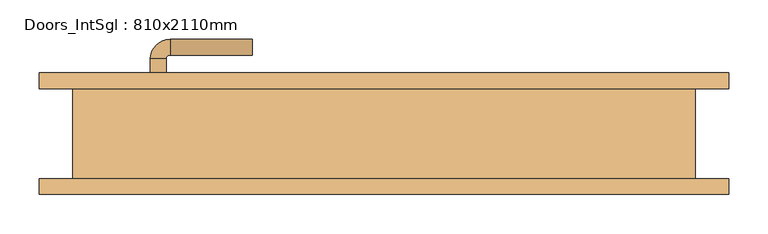
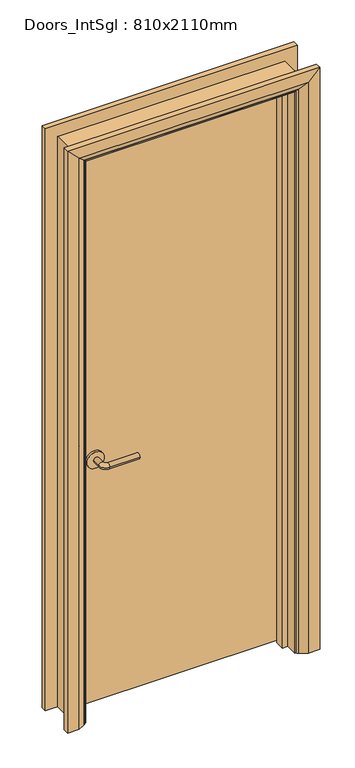
"""IFC4 building model written with IfcOpenShell, lengths in millimetres: door geometry, Doors_IntSgl : 810x2110mm."""

import ifcopenshell
import ifcopenshell.guid

model = None  # the IFC model being written
_history = None  # IfcOwnerHistory: only IFC2X3 demands one
_inside = {}  # id of a spatial element -> (the spatial element, [elements in it])
_under = {}  # id of a project, library or spatial element -> (it, [spatial elements below it])
_declared = {}  # id of a project -> (the project, [libraries it declares])
_typed = {}  # id of a type object -> (the type object, [elements of that type])
_made_of = {}  # id of a material, layer set ... -> (it, [elements and type objects made of it])


def new_model(schema):
    """Start an empty IFC model of exactly this schema.

    Asked for "IFC4X3", IfcOpenShell would pick the latest addendum, in which some entities
    have other attributes; the version numbers below select the first issue.
    IFC2X3 requires an IfcOwnerHistory on every rooted entity: one is made here for all.
    """
    global model, _history
    if schema == "IFC4X3":
        model = ifcopenshell.file(schema_version=(4, 3, 0, 0))
    else:
        model = ifcopenshell.file(schema=schema)
    _inside.clear()
    _under.clear()
    _declared.clear()
    _typed.clear()
    _made_of.clear()
    _history = None
    if model.schema == "IFC2X3":
        org = make("IfcOrganization", Name="unknown")
        user = make(
            "IfcPersonAndOrganization",
            ThePerson=make("IfcPerson", FamilyName="unknown"),
            TheOrganization=org,
        )
        app = make(
            "IfcApplication",
            ApplicationDeveloper=org,
            Version="unknown",
            ApplicationFullName="unknown",
            ApplicationIdentifier="unknown",
        )
        _history = make(
            "IfcOwnerHistory",
            OwningUser=user,
            OwningApplication=app,
            ChangeAction="ADDED",
            CreationDate=0,
        )
    return model


def make(cls, **values):
    """One entity of the class cls with the attributes given. An attribute that is None is left unset."""
    return model.create_entity(
        cls, **{name: value for name, value in values.items() if value is not None}
    )


def rooted(cls, **values):
    """An entity with a GlobalId (a new one), such as an element, a storey or a relation."""
    return make(cls, GlobalId=ifcopenshell.guid.new(), OwnerHistory=_history, **values)


def si_unit(unit_type, name, prefix=None):
    """IfcSIUnit, for example si_unit("LENGTHUNIT", "METRE", prefix="MILLI")."""
    return make("IfcSIUnit", UnitType=unit_type, Prefix=prefix, Name=name)


def assignment(units):
    """IfcUnitAssignment: the units of a project."""
    return None if units is None else make("IfcUnitAssignment", Units=units)


def point(xyz):
    """IfcCartesianPoint."""
    return None if xyz is None else make("IfcCartesianPoint", Coordinates=xyz)


def direction(xyz):
    """IfcDirection."""
    return None if xyz is None else make("IfcDirection", DirectionRatios=xyz)


def frame(location, z_axis=None, x_axis=None):
    """IfcAxis2Placement3D, a coordinate frame: its origin and axes. An axis left out is left unset."""
    return make(
        "IfcAxis2Placement3D",
        Location=point(location),
        Axis=direction(z_axis),
        RefDirection=direction(x_axis),
    )


def frame_2d(location, x_axis=None):
    """IfcAxis2Placement2D, a coordinate frame in the plane: its origin and x axis."""
    return make(
        "IfcAxis2Placement2D", Location=point(location), RefDirection=direction(x_axis)
    )


def origin():
    """The frame at (0, 0, 0) with its axes left unset."""
    return frame((0.0, 0.0, 0.0))


def place(relative_to, where):
    """IfcLocalPlacement: puts the frame where relative to a parent placement (None: the world)."""
    return make(
        "IfcLocalPlacement", PlacementRelTo=relative_to, RelativePlacement=where
    )


def context(
    kind, dimensions, precision=None, world=None, true_north=None, identifier=None
):
    """IfcGeometricRepresentationContext, for example the 3D "Model" context."""
    return make(
        "IfcGeometricRepresentationContext",
        ContextIdentifier=identifier,
        ContextType=kind,
        CoordinateSpaceDimension=dimensions,
        Precision=precision,
        WorldCoordinateSystem=world,
        TrueNorth=true_north,
    )


def project(units=None, contexts=None):
    """IfcProject with its units and contexts."""
    return rooted(
        "IfcProject",
        Name="project",
        RepresentationContexts=contexts,
        UnitsInContext=assignment(units),
    )


def spatial(cls, under=None, at=None, **own):
    """A site, building, storey or space (cls), placed at a placement, below another one or the project."""
    s = rooted(cls, ObjectPlacement=at, **own)
    if under is not None:
        _under.setdefault(under.id(), (under, []))[1].append(s)
    return s


def polyline(points):
    """IfcPolyline through the points."""
    return make("IfcPolyline", Points=[point(p) for p in points])


def circle_curve(where, radius):
    """IfcCircle in the frame where."""
    return make("IfcCircle", Position=where, Radius=radius)


def ellipse_curve(where, semi_axis1, semi_axis2):
    """IfcEllipse in the frame where."""
    return make(
        "IfcEllipse", Position=where, SemiAxis1=semi_axis1, SemiAxis2=semi_axis2
    )


def trimmed(basis, trim1, trim2, sense, master):
    """IfcTrimmedCurve: the piece of a basis curve between two trims."""
    return make(
        "IfcTrimmedCurve",
        BasisCurve=basis,
        Trim1=trim1,
        Trim2=trim2,
        SenseAgreement=sense,
        MasterRepresentation=master,
    )


def segment(curve, same_sense, transition):
    """IfcCompositeCurveSegment."""
    return make(
        "IfcCompositeCurveSegment",
        Transition=transition,
        SameSense=same_sense,
        ParentCurve=curve,
    )


def composite_curve(segments, self_intersect=None):
    """IfcCompositeCurve: segments joined end to end."""
    return make("IfcCompositeCurve", Segments=segments, SelfIntersect=self_intersect)


def outline(outer, holes=None, kind="AREA"):
    """IfcArbitraryClosedProfileDef: a profile drawn as a closed curve; with holes, ...WithVoids."""
    if holes is None:
        return make("IfcArbitraryClosedProfileDef", ProfileType=kind, OuterCurve=outer)
    return make(
        "IfcArbitraryProfileDefWithVoids",
        ProfileType=kind,
        OuterCurve=outer,
        InnerCurves=holes,
    )


def extrude(swept, where, along, depth):
    """IfcExtrudedAreaSolid: the profile swept, set in the frame where, extruded along a direction by depth."""
    return make(
        "IfcExtrudedAreaSolid",
        SweptArea=swept,
        Position=where,
        ExtrudedDirection=direction(along),
        Depth=depth,
    )


def faces_of(points, faces, orient=None, outer=None):
    """IfcFace entities. A face is a list of loops; a loop is a list of indices into points, from 0.

    orient and outer hold one flag for each loop. By default every Orientation is true, the
    first loop of a face is its IfcFaceOuterBound and the others are IfcFaceBound.
    """
    made = []
    for i, loops in enumerate(faces):
        bounds = []
        for j, loop in enumerate(loops):
            is_outer = j == 0 if outer is None else outer[i][j]
            bounds.append(
                make(
                    "IfcFaceOuterBound" if is_outer else "IfcFaceBound",
                    Bound=make("IfcPolyLoop", Polygon=[points[k] for k in loop]),
                    Orientation=True if orient is None else orient[i][j],
                )
            )
        made.append(make("IfcFace", Bounds=bounds))
    return made


def faceted_brep(points, faces, orient=None, outer=None, voids=None):
    """IfcFacetedBrep: a solid bounded by flat faces; with voids (closed shells), ...WithVoids."""
    shared = [point(p) for p in points]
    hull = make("IfcClosedShell", CfsFaces=faces_of(shared, faces, orient, outer))
    if voids is None:
        return make("IfcFacetedBrep", Outer=hull)
    return make(
        "IfcFacetedBrepWithVoids",
        Outer=hull,
        Voids=[
            make(cls, CfsFaces=faces_of(shared, fs, o, b)) for cls, fs, o, b in voids
        ],
    )


def shape(context_of_items, identifier, shape_type, items):
    """IfcShapeRepresentation: the items that make up one representation, for example the "Body"."""
    return make(
        "IfcShapeRepresentation",
        ContextOfItems=context_of_items,
        RepresentationIdentifier=identifier,
        RepresentationType=shape_type,
        Items=items,
    )


def source(mapping_origin, context_of_items, identifier, shape_type, items):
    """IfcRepresentationMap: a shape defined once, which mapped items show again and again."""
    return make(
        "IfcRepresentationMap",
        MappingOrigin=mapping_origin,
        MappedRepresentation=shape(context_of_items, identifier, shape_type, items),
    )


def transform(
    local_origin,
    x_axis=None,
    y_axis=None,
    z_axis=None,
    scale=None,
    scale2=None,
    scale3=None,
    uniform=True,
):
    """IfcCartesianTransformationOperator3D, or its non-uniform kind. x_axis, y_axis, z_axis: its Axis1, 2, 3."""
    if uniform:
        return make(
            "IfcCartesianTransformationOperator3D",
            Axis1=direction(x_axis),
            Axis2=direction(y_axis),
            LocalOrigin=point(local_origin),
            Scale=scale,
            Axis3=direction(z_axis),
        )
    return make(
        "IfcCartesianTransformationOperator3DnonUniform",
        Axis1=direction(x_axis),
        Axis2=direction(y_axis),
        LocalOrigin=point(local_origin),
        Scale=scale,
        Axis3=direction(z_axis),
        Scale2=scale2,
        Scale3=scale3,
    )


def mapped(mapping_source, mapping_target):
    """IfcMappedItem: shows the shape of a source again, moved by a transform."""
    return make(
        "IfcMappedItem", MappingSource=mapping_source, MappingTarget=mapping_target
    )


def made_of(thing, what):
    """Note that an element or type object is made of a material, layer set ...; save() writes the relation."""
    if what is not None:
        _made_of.setdefault(what.id(), (what, []))[1].append(thing)
    return thing


def element(
    cls,
    number,
    at=None,
    inside=None,
    cuts=None,
    type_object=None,
    material=None,
    context=None,
    identifier="Body",
    shape_type=None,
    held_by="IfcProductDefinitionShape",
    body=None,
    shapes=None,
    **own,
):
    """One element of the class cls, such as IfcWall. Its Tag is "e" and its number.

    at: its placement. inside: the storey or other place that contains it. cuts: it is an
    opening in that element (IfcRelVoidsElement). A single representation is given by context,
    identifier, shape_type and body (its items); several are given by shapes. held_by: the class
    of the entity that holds the representations. save() writes the other relations.
    """
    e = rooted(cls, Tag="e%d" % number, ObjectPlacement=at, **own)
    if body is not None:
        shapes = [shape(context, identifier, shape_type, body)]
    if shapes is not None:
        e.Representation = make(held_by, Representations=shapes)
    if inside is not None:
        _inside.setdefault(inside.id(), (inside, []))[1].append(e)
    if cuts is not None:
        rooted(
            "IfcRelVoidsElement", RelatingBuildingElement=cuts, RelatedOpeningElement=e
        )
    if type_object is not None:
        _typed.setdefault(type_object.id(), (type_object, []))[1].append(e)
    return made_of(e, material)


def aggregate(whole, parts):
    """IfcRelAggregates: a whole, such as a stair, and the parts it consists of."""
    return rooted("IfcRelAggregates", RelatingObject=whole, RelatedObjects=parts)


def save(model, path):
    """Write the relations noted so far, then the file.

    IfcRelAggregates (storeys below a building ...), IfcRelContainedInSpatialStructure (elements
    in a storey), IfcRelDefinesByType, IfcRelAssociatesMaterial and IfcRelDeclares: one each for
    every whole, place, type object, material and project.
    """
    for whole, parts in _under.values():
        aggregate(whole, parts)
    for where, things in _inside.values():
        rooted(
            "IfcRelContainedInSpatialStructure",
            RelatedElements=things,
            RelatingStructure=where,
        )
    for kind, things in _typed.values():
        rooted("IfcRelDefinesByType", RelatedObjects=things, RelatingType=kind)
    for what, things in _made_of.values():
        rooted("IfcRelAssociatesMaterial", RelatedObjects=things, RelatingMaterial=what)
    for by, libraries in _declared.values():
        rooted("IfcRelDeclares", RelatingContext=by, RelatedDefinitions=libraries)
    model.write(path)


def plane_surface(at):
    """IfcPlane: the flat surface through the origin of the frame at, square to its z axis."""
    return make("IfcPlane", Position=at)


def cylinder_surface(at, radius):
    """IfcCylindricalSurface: all points at the distance radius from the z axis of the frame at."""
    return make("IfcCylindricalSurface", Position=at, Radius=radius)


def revolved_surface(curve, axis_point, axis_direction):
    """IfcSurfaceOfRevolution: the curve turned about the line through axis_point along axis_direction."""
    return make(
        "IfcSurfaceOfRevolution",
        SweptCurve=make("IfcArbitraryOpenProfileDef", ProfileType="CURVE", Curve=curve),
        AxisPosition=make("IfcAxis1Placement", Location=point(axis_point), Axis=direction(axis_direction)),
    )


def advanced_brep(points, edges, surfaces, faces):
    """IfcAdvancedBrep: a solid bounded by faces that lie on surfaces and meet in shared edges.

    An edge is (start, end): straight between two places in points (the first is 0);
    or (start, end, curve); or (start, end, curve, False) where it runs against its curve.
    A face is (place in surfaces, loops), or (place, loops, False) where it looks against
    its surface's normal. A loop lists edges by number (the first is 1), with a minus sign
    where the edge is run from its end to its start. The first loop is the outer one.
    """
    corners = [point(p) for p in points]
    vertices = [make("IfcVertexPoint", VertexGeometry=c) for c in corners]
    made = []
    for start, end, *more in edges:
        made.append(
            make(
                "IfcEdgeCurve",
                EdgeStart=vertices[start],
                EdgeEnd=vertices[end],
                EdgeGeometry=more[0] if more else make("IfcPolyline", Points=[corners[start], corners[end]]),
                SameSense=more[1] if len(more) > 1 else True,
            )
        )
    hull = []
    for where, loops, *sense in faces:
        bounds = []
        for j, loop in enumerate(loops):
            ring = [make("IfcOrientedEdge", EdgeElement=made[abs(k) - 1], Orientation=k > 0) for k in loop]
            bounds.append(
                make(
                    "IfcFaceOuterBound" if j == 0 else "IfcFaceBound",
                    Bound=make("IfcEdgeLoop", EdgeList=ring),
                    Orientation=True,
                )
            )
        hull.append(make("IfcAdvancedFace", Bounds=bounds, FaceSurface=surfaces[where], SameSense=sense[0] if sense else True))
    return make("IfcAdvancedBrep", Outer=make("IfcClosedShell", CfsFaces=hull))


def doors_intsgl_810x2110mm_734bbed6(model_context):
    return source(origin(), model_context, "Body", "SolidModel", [
        advanced_brep(
        [(-298.0, 11.5, 900.0), (-278.0, 11.5, 900.0), (-278.0, -18.5, 900.0), (-298.0, -18.5, 900.0), (-273.0, -23.5, 900.0), (-273.0, -43.5, 900.0), (-168.0, -43.5, 900.0), (-168.0, -23.5, 900.0)],
        [
            (0, 1, circle_curve(frame((-288.0, 11.5, 900.0), z_axis=(0.0, 1.0, 0.0), x_axis=(1.0, 0.0, 0.0)), 10.0)),
            (1, 0, circle_curve(frame((-288.0, 11.5, 900.0), z_axis=(0.0, 1.0, 0.0), x_axis=(1.0, 0.0, 0.0)), 10.0)),
            (1, 2),
            (2, 3, circle_curve(frame((-288.0, -18.5, 900.0), z_axis=(0.0, 1.0, 0.0), x_axis=(1.0, 0.0, 0.0)), 10.0)),
            (3, 0),
            (3, 2, circle_curve(frame((-288.0, -18.5, 900.0), z_axis=(0.0, 1.0, 0.0), x_axis=(1.0, 0.0, 0.0)), 10.0)),
            (4, 5, circle_curve(frame((-273.0, -33.5, 900.0), z_axis=(-1.0, 0.0, 0.0), x_axis=(0.0, 1.0, 0.0)), 10.0)),
            (5, 3, circle_curve(frame((-273.0, -18.5, 900.0), z_axis=(0.0, 0.0, -1.0), x_axis=(-1.0, 0.0, 0.0)), 25.0)),
            (2, 4, circle_curve(frame((-273.0, -18.5, 900.0), z_axis=(0.0, 0.0, 1.0), x_axis=(-1.0, 0.0, 0.0)), 5.0)),
            (5, 4, circle_curve(frame((-273.0, -33.5, 900.0), z_axis=(-1.0, 0.0, 0.0), x_axis=(0.0, 1.0, 0.0)), 10.0)),
            (6, 7, circle_curve(frame((-168.0, -33.5, 900.0), z_axis=(1.0, 0.0, 0.0), x_axis=(0.0, 1.0, 0.0)), 10.0)),
            (7, 6, circle_curve(frame((-168.0, -33.5, 900.0), z_axis=(1.0, 0.0, 0.0), x_axis=(0.0, 1.0, 0.0)), 10.0)),
            (4, 7),
            (6, 5),
        ],
        [
            plane_surface(frame((-288.0, 11.5, 900.0), z_axis=(0.0, 1.0, 0.0), x_axis=(0.0, 0.0, 1.0))),
            cylinder_surface(frame((-288.0, 11.5, 900.0), z_axis=(0.0, 1.0, 0.0), x_axis=(1.0, 0.0, 0.0)), 10.0),
            revolved_surface(trimmed(ellipse_curve(frame((-288.0, -18.5, 900.0), z_axis=(0.0, -1.0, 0.0), x_axis=(1.0, 0.0, 0.0)), 10.0, 10.0), [point((-298.0, -18.5, 900.0))], [point((-278.0, -18.5, 900.0))], True, "CARTESIAN"), (-273.0, -18.5, 900.0), (0.0, 0.0, -1.0)),
            revolved_surface(trimmed(ellipse_curve(frame((-288.0, -18.5, 900.0), z_axis=(0.0, -1.0, 0.0), x_axis=(1.0, 0.0, 0.0)), 10.0, 10.0), [point((-278.0, -18.5, 900.0))], [point((-298.0, -18.5, 900.0))], True, "CARTESIAN"), (-273.0, -18.5, 900.0), (0.0, 0.0, -1.0)),
            plane_surface(frame((-168.0, -33.5, 900.0), z_axis=(1.0, 0.0, 0.0), x_axis=(0.0, 0.0, 1.0))),
            cylinder_surface(frame((-273.0, -33.5, 900.0), z_axis=(-1.0, 0.0, 0.0), x_axis=(0.0, 1.0, 0.0)), 10.0),
        ],
        [
            (0, [[1, 2]]),
            (1, [[3, 4, 5, -2]]),
            (1, [[-5, 6, -3, -1]]),
            (2, [[7, 8, -4, 9]]),
            (3, [[10, -9, -6, -8]]),
            (4, [[11, 12]]),
            (5, [[13, -11, 14, -7]]),
            (5, [[-14, -12, -13, -10]]),
        ],
    ),
        extrude(outline(composite_curve([segment(trimmed(circle_curve(frame_2d((900.0, -290.5)), 30.0), [point((900.0, -320.5))], [point((900.0, -260.5))], False, "CARTESIAN"), True, "CONTINUOUS"), segment(trimmed(circle_curve(frame_2d((900.0, -290.5)), 30.0), [point((900.0, -260.5))], [point((900.0, -320.5))], False, "CARTESIAN"), True, "CONTINUOUS")], self_intersect=False)), frame((0.0, 11.5, 0.0), z_axis=(0.0, 1.0, 0.0), x_axis=(0.0, 0.0, 1.0)), (0.0, 0.0, 1.0), 8.0),
        advanced_brep(
        [(-298.0, 65.5, 900.0), (-278.0, 65.5, 900.0), (-298.0, 95.5, 900.0), (-278.0, 95.5, 900.0), (-273.0, 100.5, 900.0), (-273.0, 120.5, 900.0), (-168.0, 120.5, 900.0), (-168.0, 100.5, 900.0)],
        [
            (0, 1, circle_curve(frame((-288.0, 65.5, 900.0), z_axis=(0.0, -1.0, 0.0), x_axis=(1.0, 0.0, 0.0)), 10.0)),
            (1, 0, circle_curve(frame((-288.0, 65.5, 900.0), z_axis=(0.0, -1.0, 0.0), x_axis=(1.0, 0.0, 0.0)), 10.0)),
            (0, 2),
            (2, 3, circle_curve(frame((-288.0, 95.5, 900.0), z_axis=(0.0, -1.0, 0.0), x_axis=(1.0, 0.0, 0.0)), 10.0)),
            (3, 1),
            (3, 2, circle_curve(frame((-288.0, 95.5, 900.0), z_axis=(0.0, -1.0, 0.0), x_axis=(1.0, 0.0, 0.0)), 10.0)),
            (4, 3, circle_curve(frame((-273.0, 95.5, 900.0), z_axis=(0.0, 0.0, 1.0), x_axis=(-1.0, 0.0, 0.0)), 5.0)),
            (2, 5, circle_curve(frame((-273.0, 95.5, 900.0), z_axis=(0.0, 0.0, -1.0), x_axis=(-1.0, 0.0, 0.0)), 25.0)),
            (5, 4, circle_curve(frame((-273.0, 110.5, 900.0), z_axis=(-1.0, 0.0, 0.0), x_axis=(0.0, -1.0, 0.0)), 10.0)),
            (4, 5, circle_curve(frame((-273.0, 110.5, 900.0), z_axis=(-1.0, 0.0, 0.0), x_axis=(0.0, -1.0, 0.0)), 10.0)),
            (6, 7, circle_curve(frame((-168.0, 110.5, 900.0), z_axis=(1.0, 0.0, 0.0), x_axis=(0.0, -1.0, 0.0)), 10.0)),
            (7, 6, circle_curve(frame((-168.0, 110.5, 900.0), z_axis=(1.0, 0.0, 0.0), x_axis=(0.0, -1.0, 0.0)), 10.0)),
            (5, 6),
            (7, 4),
        ],
        [
            plane_surface(frame((-288.0, 65.5, 900.0), z_axis=(0.0, -1.0, 0.0), x_axis=(0.0, 0.0, 1.0))),
            cylinder_surface(frame((-288.0, 65.5, 900.0), z_axis=(0.0, -1.0, 0.0), x_axis=(1.0, 0.0, 0.0)), 10.0),
            revolved_surface(trimmed(ellipse_curve(frame((-288.0, 95.5, 900.0), z_axis=(0.0, -1.0, 0.0), x_axis=(1.0, 0.0, 0.0)), 10.0, 10.0), [point((-298.0, 95.5, 900.0))], [point((-278.0, 95.5, 900.0))], True, "CARTESIAN"), (-273.0, 95.5, 900.0), (0.0, 0.0, -1.0)),
            revolved_surface(trimmed(ellipse_curve(frame((-288.0, 95.5, 900.0), z_axis=(0.0, -1.0, 0.0), x_axis=(1.0, 0.0, 0.0)), 10.0, 10.0), [point((-278.0, 95.5, 900.0))], [point((-298.0, 95.5, 900.0))], True, "CARTESIAN"), (-273.0, 95.5, 900.0), (0.0, 0.0, -1.0)),
            plane_surface(frame((-168.0, 110.5, 900.0), z_axis=(1.0, 0.0, 0.0), x_axis=(0.0, 0.0, 1.0))),
            cylinder_surface(frame((-273.0, 110.5, 900.0), z_axis=(-1.0, 0.0, 0.0), x_axis=(0.0, -1.0, 0.0)), 10.0),
        ],
        [
            (0, [[1, 2]]),
            (1, [[-1, 3, 4, 5]]),
            (1, [[-2, -5, 6, -3]]),
            (2, [[7, -4, 8, 9]]),
            (3, [[-8, -6, -7, 10]]),
            (4, [[11, 12]]),
            (5, [[-9, 13, -12, 14]]),
            (5, [[-10, -14, -11, -13]]),
        ],
    ),
        extrude(outline(composite_curve([segment(trimmed(circle_curve(frame_2d((900.0, -290.5)), 30.0), [point((900.0, -320.5))], [point((900.0, -260.5))], False, "CARTESIAN"), True, "CONTINUOUS"), segment(trimmed(circle_curve(frame_2d((900.0, -290.5)), 30.0), [point((900.0, -260.5))], [point((900.0, -320.5))], False, "CARTESIAN"), True, "CONTINUOUS")], self_intersect=False)), frame((0.0, 57.5, 0.0), z_axis=(0.0, 1.0, 0.0), x_axis=(0.0, 0.0, 1.0)), (0.0, 0.0, 1.0), 8.0),
        extrude(outline(polyline([(363.0, 19.5), (-363.0, 19.5), (-363.0, 57.5), (363.0, 57.5), (363.0, 19.5)])), frame((0.0, 0.0, 8.0), z_axis=(0.0, 0.0, 1.0), x_axis=(1.0, 0.0, 0.0)), (0.0, 0.0, 1.0), 2060.0),
        advanced_brep(
        [(440.0, 77.5, 0.0), (440.0, 57.5, 0.0), (370.0, 57.5, 0.0), (374.0, 63.5, 0.0), (400.0, 77.5, 0.0), (440.0, 77.5, 2145.0), (440.0, 57.5, 2145.0), (-440.0, 57.5, 2145.0), (-440.0, 57.5, 0.0), (-370.0, 57.5, 0.0), (-370.0, 57.5, 2075.0), (370.0, 57.5, 2075.0), (374.0, 63.5, 2079.0), (400.0, 77.5, 2105.0), (-400.0, 77.5, 2105.0), (-400.0, 77.5, 0.0), (-440.0, 77.5, 0.0), (-440.0, 77.5, 2145.0), (-374.0, 63.5, 2079.0), (-374.0, 63.5, 0.0)],
        [
            (0, 1),
            (1, 2),
            (2, 3, circle_curve(frame((378.0, 56.5, 0.0), z_axis=(0.0, 0.0, -1.0), x_axis=(1.0, 0.0, 0.0)), 8.0622577)),
            (3, 4),
            (4, 0),
            (0, 5),
            (5, 6),
            (6, 1),
            (6, 7),
            (7, 8),
            (8, 9),
            (9, 10),
            (10, 11),
            (11, 2),
            (11, 12, ellipse_curve(frame((378.0, 56.5, 2083.0), z_axis=(0.7071067811865475, 0.0, -0.7071067811865475), x_axis=(-0.7071067811865474, 0.0, -0.7071067811865476)), 11.4017543, 8.0622577)),
            (12, 3),
            (12, 13),
            (13, 4),
            (13, 14),
            (14, 15),
            (15, 16),
            (16, 17),
            (17, 5),
            (17, 7),
            (10, 18, ellipse_curve(frame((-378.0, 56.5, 2083.0), z_axis=(0.7071067811865475, 0.0, 0.7071067811865475), x_axis=(0.7071067811865476, 0.0, -0.7071067811865474)), 11.4017543, 8.0622577)),
            (18, 12),
            (18, 14),
            (15, 19),
            (19, 9, circle_curve(frame((-378.0, 56.5, 0.0), z_axis=(0.0, 0.0, -1.0), x_axis=(-1.0, 0.0, 0.0)), 8.0622577)),
            (8, 16),
            (19, 18),
        ],
        [
            plane_surface(frame((370.0, 57.5, 0.0), z_axis=(0.0, 0.0, -1.0), x_axis=(0.0, -1.0, 0.0))),
            plane_surface(frame((440.0, 77.5, 0.0), z_axis=(1.0, 0.0, 0.0), x_axis=(0.0, 0.0, 1.0))),
            plane_surface(frame((440.0, 57.5, 0.0), z_axis=(0.0, -1.0, 0.0), x_axis=(0.0, 0.0, 1.0))),
            cylinder_surface(frame((378.0, 56.5, 0.0), z_axis=(0.0, 0.0, -1.0), x_axis=(1.0, 0.0, 0.0)), 8.0622577),
            plane_surface(frame((374.0, 63.5, 0.0), z_axis=(-0.4740998230350126, 0.880471099922178, 0.0), x_axis=(0.0, 0.0, 1.0))),
            plane_surface(frame((400.0, 77.5, 0.0), z_axis=(0.0, 1.0, 0.0), x_axis=(0.0, 0.0, 1.0))),
            plane_surface(frame((440.0, 77.5, 2145.0), z_axis=(0.0, 0.0, 1.0), x_axis=(-1.0, 0.0, 0.0))),
            cylinder_surface(frame((370.0, 56.5, 2083.0), z_axis=(1.0, 0.0, 0.0), x_axis=(0.0, 0.0, 1.0)), 8.0622577),
            plane_surface(frame((374.0, 63.5, 2079.0), z_axis=(0.0, 0.8804710999221764, -0.4740998230350154), x_axis=(-1.0, 0.0, 0.0))),
            plane_surface(frame((-370.0, 57.5, 0.0), z_axis=(0.0, 0.0, -1.0), x_axis=(0.0, -1.0, 0.0))),
            plane_surface(frame((-440.0, 77.5, 2145.0), z_axis=(-1.0, 0.0, 0.0), x_axis=(0.0, 0.0, -1.0))),
            cylinder_surface(frame((-378.0, 56.5, 2075.0), z_axis=(0.0, 0.0, 1.0), x_axis=(-1.0, 0.0, 0.0)), 8.0622577),
            plane_surface(frame((-374.0, 63.5, 2079.0), z_axis=(0.47409982303501824, 0.8804710999221749, 0.0), x_axis=(0.0, 0.0, -1.0))),
        ],
        [
            (0, [[1, 2, 3, 4, 5]]),
            (1, [[-1, 6, 7, 8]]),
            (2, [[-2, -8, 9, 10, 11, 12, 13, 14]]),
            (3, [[-3, -14, 15, 16]]),
            (4, [[-4, -16, 17, 18]]),
            (5, [[-5, -18, 19, 20, 21, 22, 23, -6]]),
            (6, [[-7, -23, 24, -9]]),
            (7, [[-15, -13, 25, 26]]),
            (8, [[-17, -26, 27, -19]]),
            (9, [[-21, 28, 29, -11, 30]]),
            (10, [[-24, -22, -30, -10]]),
            (11, [[-25, -12, -29, 31]]),
            (12, [[-27, -31, -28, -20]]),
        ],
    ),
        extrude(outline(polyline([(0.0, -365.0), (0.0, -346.0), (2051.0, -346.0), (2051.0, 346.0), (0.0, 346.0), (0.0, 365.0), (2070.0, 365.0), (2070.0, -365.0), (0.0, -365.0)])), frame((0.0, -14.5, 0.0), z_axis=(0.0, 1.0, 0.0), x_axis=(0.0, 0.0, 1.0)), (0.0, 0.0, 1.0), 32.0),
        advanced_brep(
        [(-440.0, -77.5, 0.0), (-440.0, -57.5, 0.0), (-370.0, -57.5, 0.0), (-374.0, -63.5, 0.0), (-400.0, -77.5, 0.0), (-440.0, -77.5, 2145.0), (-440.0, -57.5, 2145.0), (-370.0, -57.5, 2075.0), (-374.0, -63.5, 2079.0), (-400.0, -77.5, 2105.0), (440.0, -77.5, 2145.0), (440.0, -57.5, 2145.0), (370.0, -57.5, 2075.0), (374.0, -63.5, 2079.0), (400.0, -77.5, 2105.0), (440.0, -77.5, 0.0), (400.0, -77.5, 0.0), (374.0, -63.5, 0.0), (370.0, -57.5, 0.0), (440.0, -57.5, 0.0)],
        [
            (0, 1),
            (1, 2),
            (2, 3, circle_curve(frame((-378.0, -56.5, 0.0), z_axis=(0.0, 0.0, -1.0), x_axis=(-1.0, 0.0, 0.0)), 8.0622577)),
            (3, 4),
            (4, 0),
            (0, 5),
            (5, 6),
            (6, 1),
            (6, 7),
            (7, 2),
            (7, 8, ellipse_curve(frame((-378.0, -56.5, 2083.0), z_axis=(-0.7071067811865475, 0.0, -0.7071067811865475), x_axis=(0.7071067811865474, 0.0, -0.7071067811865476)), 11.4017543, 8.0622577)),
            (8, 3),
            (8, 9),
            (9, 4),
            (9, 5),
            (5, 10),
            (10, 11),
            (11, 6),
            (11, 12),
            (12, 7),
            (12, 13, ellipse_curve(frame((378.0, -56.5, 2083.0), z_axis=(-0.7071067811865475, 0.0, 0.7071067811865475), x_axis=(-0.7071067811865476, 0.0, -0.7071067811865474)), 11.4017543, 8.0622577)),
            (13, 8),
            (13, 14),
            (14, 9),
            (14, 10),
            (15, 16),
            (16, 17),
            (17, 18, circle_curve(frame((378.0, -56.5, 0.0), z_axis=(0.0, 0.0, -1.0), x_axis=(1.0, 0.0, 0.0)), 8.0622577)),
            (18, 19),
            (19, 15),
            (10, 15),
            (19, 11),
            (18, 12),
            (17, 13),
            (16, 14),
        ],
        [
            plane_surface(frame((-370.0, -130.3010989, 0.0), z_axis=(0.0, 0.0, -1.0), x_axis=(1.0, 0.0, 0.0))),
            plane_surface(frame((-440.0, -77.5, 0.0), z_axis=(-1.0, 0.0, 0.0), x_axis=(0.0, 0.0, 1.0))),
            plane_surface(frame((-440.0, -57.5, 0.0), z_axis=(0.0, 1.0, 0.0), x_axis=(0.0, 0.0, 1.0))),
            cylinder_surface(frame((-378.0, -56.5, 0.0), z_axis=(0.0, 0.0, -1.0), x_axis=(-1.0, 0.0, 0.0)), 8.0622577),
            plane_surface(frame((-374.0, -63.5, 0.0), z_axis=(0.4740998230350183, -0.8804710999221749, 0.0), x_axis=(0.0, 0.0, 1.0))),
            plane_surface(frame((-400.0, -77.5, 0.0), z_axis=(0.0, -1.0, 0.0), x_axis=(0.0, 0.0, 1.0))),
            plane_surface(frame((-440.0, -77.5, 2145.0), z_axis=(0.0, 0.0, 1.0), x_axis=(1.0, 0.0, 0.0))),
            plane_surface(frame((-440.0, -57.5, 2145.0), z_axis=(0.0, 1.0, 0.0), x_axis=(1.0, 0.0, 0.0))),
            cylinder_surface(frame((-370.0, -56.5, 2083.0), z_axis=(-1.0, 0.0, 0.0), x_axis=(0.0, 0.0, 1.0)), 8.0622577),
            plane_surface(frame((-374.0, -63.5, 2079.0), z_axis=(0.0, -0.8804710999221749, -0.4740998230350183), x_axis=(1.0, 0.0, 0.0))),
            plane_surface(frame((-400.0, -77.5, 2105.0), z_axis=(0.0, -1.0, 0.0), x_axis=(1.0, 0.0, 0.0))),
            plane_surface(frame((370.0, -130.3010989, 0.0), z_axis=(0.0, 0.0, -1.0), x_axis=(-1.0, 0.0, 0.0))),
            plane_surface(frame((440.0, -77.5, 2145.0), z_axis=(1.0, 0.0, 0.0), x_axis=(0.0, 0.0, -1.0))),
            plane_surface(frame((440.0, -57.5, 2145.0), z_axis=(0.0, 1.0, 0.0), x_axis=(0.0, 0.0, -1.0))),
            cylinder_surface(frame((378.0, -56.5, 2075.0), z_axis=(0.0, 0.0, 1.0), x_axis=(1.0, 0.0, 0.0)), 8.0622577),
            plane_surface(frame((374.0, -63.5, 2079.0), z_axis=(-0.4740998230350183, -0.8804710999221749, 0.0), x_axis=(0.0, 0.0, -1.0))),
            plane_surface(frame((400.0, -77.5, 2105.0), z_axis=(0.0, -1.0, 0.0), x_axis=(0.0, 0.0, -1.0))),
        ],
        [
            (0, [[1, 2, 3, 4, 5]]),
            (1, [[-1, 6, 7, 8]]),
            (2, [[-2, -8, 9, 10]]),
            (3, [[-3, -10, 11, 12]]),
            (4, [[-4, -12, 13, 14]]),
            (5, [[-5, -14, 15, -6]]),
            (6, [[-7, 16, 17, 18]]),
            (7, [[-9, -18, 19, 20]]),
            (8, [[-11, -20, 21, 22]]),
            (9, [[-13, -22, 23, 24]]),
            (10, [[-15, -24, 25, -16]]),
            (11, [[26, 27, 28, 29, 30]]),
            (12, [[-17, 31, -30, 32]]),
            (13, [[-19, -32, -29, 33]]),
            (14, [[-21, -33, -28, 34]]),
            (15, [[-23, -34, -27, 35]]),
            (16, [[-25, -35, -26, -31]]),
        ],
    ),
        faceted_brep([(-365.0, 57.5, 0.0), (-365.0, -57.5, 0.0), (-397.0, -57.5, 0.0), (-397.0, 57.5, 0.0), (-365.0, 57.5, 2070.0), (-365.0, -57.5, 2070.0), (-397.0, -57.5, 2102.0), (-397.0, 57.5, 2102.0), (365.0, 57.5, 2070.0), (365.0, -57.5, 2070.0), (397.0, -57.5, 2102.0), (397.0, 57.5, 2102.0), (365.0, 57.5, 0.0), (397.0, 57.5, 0.0), (397.0, -57.5, 0.0), (365.0, -57.5, 0.0)], [[[0, 1, 2, 3]], [[1, 0, 4, 5]], [[2, 1, 5, 6]], [[3, 2, 6, 7]], [[0, 3, 7, 4]], [[5, 4, 8, 9]], [[6, 5, 9, 10]], [[7, 6, 10, 11]], [[4, 7, 11, 8]], [[12, 13, 14, 15]], [[9, 8, 12, 15]], [[10, 9, 15, 14]], [[11, 10, 14, 13]], [[8, 11, 13, 12]]]),
    ])


if __name__ == "__main__":
    model = new_model("IFC4")
    model_context = context("Model", 3, world=origin())
    ifc_project = project(units=[si_unit("LENGTHUNIT", "METRE", prefix="MILLI")], contexts=[model_context])
    site = spatial("IfcSite", under=ifc_project)
    building = spatial("IfcBuilding", under=site)
    placement = place(None, origin())
    doors_intsgl_810x2110mm_shape = doors_intsgl_810x2110mm_734bbed6(model_context)
    element("IfcDoor", 1, ObjectType="Doors_IntSgl : 810x2110mm", at=placement, inside=building, context=model_context, shape_type="MappedRepresentation", body=[
        mapped(doors_intsgl_810x2110mm_shape, transform((0.0, 0.0, 0.0), x_axis=(1.0, 0.0, 0.0), y_axis=(0.0, 1.0, 0.0), z_axis=(0.0, 0.0, 1.0))),
    ])
    save(model, "model.ifc")

# Revit data of these elements
# Type "Doors_IntSgl : 810x2110mm"
#   Construction Type Id = "MDOOR"
#   Type Mark = "42"
#   Type Comments = "Internal Single"
#   Operation = "SingleSwingRight"
#   Manufacturer = "Revit"
#   Keynote = "L20"
#   Description = "Internal Single Door"
#   Analytic Construction = "Metal"
#   UnderCut = 8 mm
#   Tolerance = 2 mm
#   Thickness = 38 mm
#   Thermal Resistance (R) = 0.270117 (m²·K)/W
#   Structural Tolerance = 8 mm
#   StopDepth = 32 mm
#   Stop Thickness = 19 mm
#   Rough Width = 810 mm
#   Rough Height = 2110 mm
#   Height to Top Lock Rail = 1000 mm
#   Heat Transfer Coefficient (U) = 3.7021 W/(m²·K)
#   Handle Z Distance = 900 mm
#   Handle X Distance = 75 mm
#   Frame Thickness = 32 mm
#   Door Panel Width = 726 mm
#   Door Panel Thickness = 38 mm
#   Door Panel Offset = 0 mm
#   Height = 2110 mm
#   Width = 810 mm
#   Door Panel Height = 2060 mm
#   Architrave Setback = 5 mm
#   Define Thermal Properties by = 1
#   Vis - Ironmongery = yes
#   Material Ironmongery = Door - Handle
#   Material Frame = Door - Frame/Mullion (1)
#   Material Door = Door - Panel
#   Material Architrave = Door - Architrave
#   Visual Light Transmittance = 0
#   Solar Heat Gain Coefficient = 0
#   Function = (empty or 0)
#   Wall Closure = (empty or 0)
# Element 1 (IfcDoor, "Doors_IntSgl : 810x2110mm")
#   Materials on its faces: "Door - Architrave", "Door - Handle", "Door - Frame/Mullion (1)", "Door - Panel"
# Materials
#   "Door - Handle": class "Miscellaneous", colour RGB 0 0 0, transparency 0, Keynote = "P21", Cost = 0
#   "Door - Frame/Mullion (1)": class "Wood", colour RGB 212 179 113, transparency 0, Keynote = "L20", Cost = 0
#   "Door - Panel": class "Wood", colour RGB 210 159 95, transparency 0, Keynote = "L20", Cost = 0
#   "Door - Architrave": class "Wood", colour RGB 154 90 5, transparency 0, Keynote = "P20", Cost = 0
